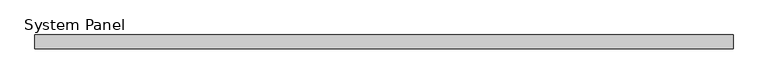
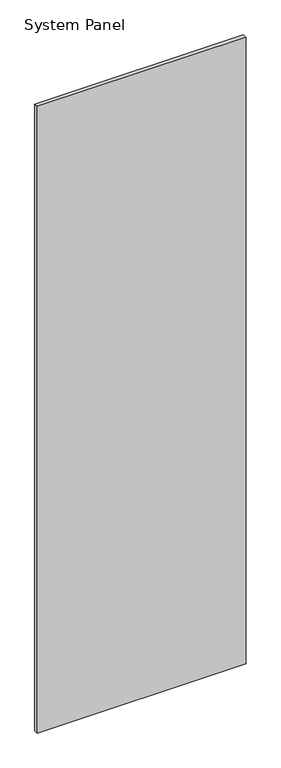
"""IFC4 building model written with IfcOpenShell, lengths in millimetres: plate geometry, System Panel : WWm-Glass-20mm-10mmOffset."""

from ifc_helpers import new_model, si_unit, origin, origin_with_axes, place, context, project, spatial, polyline, outline, extrude, source, transform, mapped, element, save


def system_panel_8548a333(model_context):
    return source(origin(), model_context, "Body", "SweptSolid", [
        extrude(outline(polyline([(512.5, 0.0), (-512.5, 0.0), (-512.5, 20.0), (512.5, 20.0), (512.5, 0.0)])), origin_with_axes(), (0.0, 0.0, 1.0), 3250.0),
    ])


if __name__ == "__main__":
    model = new_model("IFC4")
    model_context = context("Model", 3, world=origin())
    ifc_project = project(units=[si_unit("LENGTHUNIT", "METRE", prefix="MILLI")], contexts=[model_context])
    site = spatial("IfcSite", under=ifc_project)
    building = spatial("IfcBuilding", under=site)
    placement = place(None, origin())
    system_panel_shape = system_panel_8548a333(model_context)
    element("IfcPlate", 1, ObjectType="System Panel : WWm-Glass-20mm-10mmOffset", at=placement, inside=building, context=model_context, shape_type="MappedRepresentation", body=[
        mapped(system_panel_shape, transform((0.0, 0.0, 0.0), x_axis=(1.0, 0.0, 0.0), y_axis=(0.0, 1.0, 0.0), z_axis=(0.0, 0.0, 1.0))),
    ])
    save(model, "model.ifc")

# Revit data of these elements
# Type "System Panel : WWm-Glass-20mm-10mmOffset"
#   Finish = ""
# Element 1 (IfcPlate, "System Panel : WWm-Glass-20mm-10mmOffset")
#   Materials on its faces: "WW-EC-GL-Storefront"
# Materials
#   "WW-EC-GL-Storefront": class "Glass", colour RGB 236 240 239, transparency 0.85, Description = "Storefront Glass", Cost = 0
